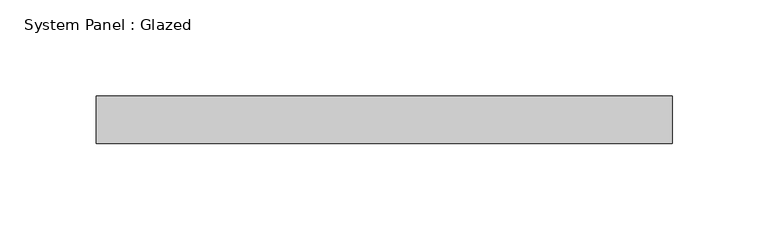
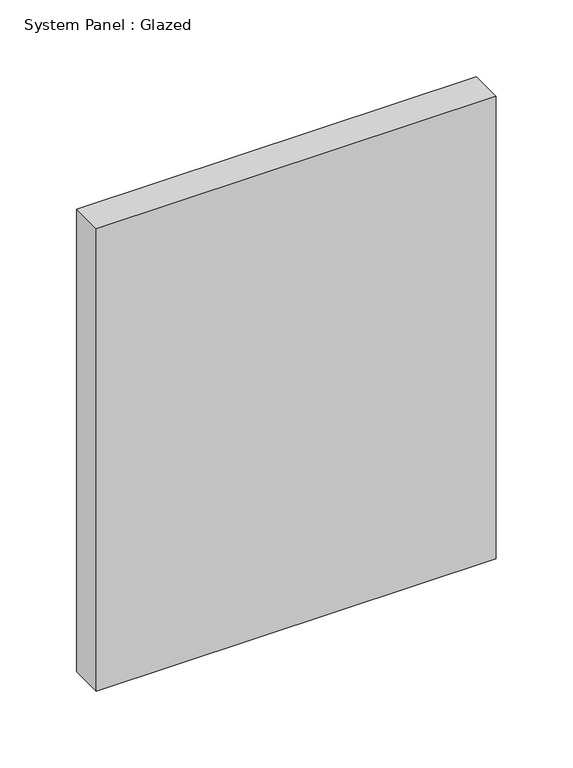
"""IFC4 building model written with IfcOpenShell, lengths in millimetres: plate geometry, System Panel : Glazed."""

import ifcopenshell
import ifcopenshell.guid

model = None  # the IFC model being written
_history = None  # IfcOwnerHistory: only IFC2X3 demands one
_inside = {}  # id of a spatial element -> (the spatial element, [elements in it])
_under = {}  # id of a project, library or spatial element -> (it, [spatial elements below it])
_declared = {}  # id of a project -> (the project, [libraries it declares])
_typed = {}  # id of a type object -> (the type object, [elements of that type])
_made_of = {}  # id of a material, layer set ... -> (it, [elements and type objects made of it])


def new_model(schema):
    """Start an empty IFC model of exactly this schema.

    Asked for "IFC4X3", IfcOpenShell would pick the latest addendum, in which some entities
    have other attributes; the version numbers below select the first issue.
    IFC2X3 requires an IfcOwnerHistory on every rooted entity: one is made here for all.
    """
    global model, _history
    if schema == "IFC4X3":
        model = ifcopenshell.file(schema_version=(4, 3, 0, 0))
    else:
        model = ifcopenshell.file(schema=schema)
    _inside.clear()
    _under.clear()
    _declared.clear()
    _typed.clear()
    _made_of.clear()
    _history = None
    if model.schema == "IFC2X3":
        org = make("IfcOrganization", Name="unknown")
        user = make(
            "IfcPersonAndOrganization",
            ThePerson=make("IfcPerson", FamilyName="unknown"),
            TheOrganization=org,
        )
        app = make(
            "IfcApplication",
            ApplicationDeveloper=org,
            Version="unknown",
            ApplicationFullName="unknown",
            ApplicationIdentifier="unknown",
        )
        _history = make(
            "IfcOwnerHistory",
            OwningUser=user,
            OwningApplication=app,
            ChangeAction="ADDED",
            CreationDate=0,
        )
    return model


def make(cls, **values):
    """One entity of the class cls with the attributes given. An attribute that is None is left unset."""
    return model.create_entity(
        cls, **{name: value for name, value in values.items() if value is not None}
    )


def rooted(cls, **values):
    """An entity with a GlobalId (a new one), such as an element, a storey or a relation."""
    return make(cls, GlobalId=ifcopenshell.guid.new(), OwnerHistory=_history, **values)


def si_unit(unit_type, name, prefix=None):
    """IfcSIUnit, for example si_unit("LENGTHUNIT", "METRE", prefix="MILLI")."""
    return make("IfcSIUnit", UnitType=unit_type, Prefix=prefix, Name=name)


def assignment(units):
    """IfcUnitAssignment: the units of a project."""
    return None if units is None else make("IfcUnitAssignment", Units=units)


def point(xyz):
    """IfcCartesianPoint."""
    return None if xyz is None else make("IfcCartesianPoint", Coordinates=xyz)


def direction(xyz):
    """IfcDirection."""
    return None if xyz is None else make("IfcDirection", DirectionRatios=xyz)


def frame(location, z_axis=None, x_axis=None):
    """IfcAxis2Placement3D, a coordinate frame: its origin and axes. An axis left out is left unset."""
    return make(
        "IfcAxis2Placement3D",
        Location=point(location),
        Axis=direction(z_axis),
        RefDirection=direction(x_axis),
    )


def origin():
    """The frame at (0, 0, 0) with its axes left unset."""
    return frame((0.0, 0.0, 0.0))


def origin_with_axes():
    """The frame at (0, 0, 0) with the z axis (0, 0, 1) and the x axis (1, 0, 0) written out."""
    return frame((0.0, 0.0, 0.0), z_axis=(0.0, 0.0, 1.0), x_axis=(1.0, 0.0, 0.0))


def place(relative_to, where):
    """IfcLocalPlacement: puts the frame where relative to a parent placement (None: the world)."""
    return make(
        "IfcLocalPlacement", PlacementRelTo=relative_to, RelativePlacement=where
    )


def context(
    kind, dimensions, precision=None, world=None, true_north=None, identifier=None
):
    """IfcGeometricRepresentationContext, for example the 3D "Model" context."""
    return make(
        "IfcGeometricRepresentationContext",
        ContextIdentifier=identifier,
        ContextType=kind,
        CoordinateSpaceDimension=dimensions,
        Precision=precision,
        WorldCoordinateSystem=world,
        TrueNorth=true_north,
    )


def project(units=None, contexts=None):
    """IfcProject with its units and contexts."""
    return rooted(
        "IfcProject",
        Name="project",
        RepresentationContexts=contexts,
        UnitsInContext=assignment(units),
    )


def spatial(cls, under=None, at=None, **own):
    """A site, building, storey or space (cls), placed at a placement, below another one or the project."""
    s = rooted(cls, ObjectPlacement=at, **own)
    if under is not None:
        _under.setdefault(under.id(), (under, []))[1].append(s)
    return s


def polyline(points):
    """IfcPolyline through the points."""
    return make("IfcPolyline", Points=[point(p) for p in points])


def outline(outer, holes=None, kind="AREA"):
    """IfcArbitraryClosedProfileDef: a profile drawn as a closed curve; with holes, ...WithVoids."""
    if holes is None:
        return make("IfcArbitraryClosedProfileDef", ProfileType=kind, OuterCurve=outer)
    return make(
        "IfcArbitraryProfileDefWithVoids",
        ProfileType=kind,
        OuterCurve=outer,
        InnerCurves=holes,
    )


def extrude(swept, where, along, depth):
    """IfcExtrudedAreaSolid: the profile swept, set in the frame where, extruded along a direction by depth."""
    return make(
        "IfcExtrudedAreaSolid",
        SweptArea=swept,
        Position=where,
        ExtrudedDirection=direction(along),
        Depth=depth,
    )


def shape(context_of_items, identifier, shape_type, items):
    """IfcShapeRepresentation: the items that make up one representation, for example the "Body"."""
    return make(
        "IfcShapeRepresentation",
        ContextOfItems=context_of_items,
        RepresentationIdentifier=identifier,
        RepresentationType=shape_type,
        Items=items,
    )


def source(mapping_origin, context_of_items, identifier, shape_type, items):
    """IfcRepresentationMap: a shape defined once, which mapped items show again and again."""
    return make(
        "IfcRepresentationMap",
        MappingOrigin=mapping_origin,
        MappedRepresentation=shape(context_of_items, identifier, shape_type, items),
    )


def transform(
    local_origin,
    x_axis=None,
    y_axis=None,
    z_axis=None,
    scale=None,
    scale2=None,
    scale3=None,
    uniform=True,
):
    """IfcCartesianTransformationOperator3D, or its non-uniform kind. x_axis, y_axis, z_axis: its Axis1, 2, 3."""
    if uniform:
        return make(
            "IfcCartesianTransformationOperator3D",
            Axis1=direction(x_axis),
            Axis2=direction(y_axis),
            LocalOrigin=point(local_origin),
            Scale=scale,
            Axis3=direction(z_axis),
        )
    return make(
        "IfcCartesianTransformationOperator3DnonUniform",
        Axis1=direction(x_axis),
        Axis2=direction(y_axis),
        LocalOrigin=point(local_origin),
        Scale=scale,
        Axis3=direction(z_axis),
        Scale2=scale2,
        Scale3=scale3,
    )


def mapped(mapping_source, mapping_target):
    """IfcMappedItem: shows the shape of a source again, moved by a transform."""
    return make(
        "IfcMappedItem", MappingSource=mapping_source, MappingTarget=mapping_target
    )


def made_of(thing, what):
    """Note that an element or type object is made of a material, layer set ...; save() writes the relation."""
    if what is not None:
        _made_of.setdefault(what.id(), (what, []))[1].append(thing)
    return thing


def element(
    cls,
    number,
    at=None,
    inside=None,
    cuts=None,
    type_object=None,
    material=None,
    context=None,
    identifier="Body",
    shape_type=None,
    held_by="IfcProductDefinitionShape",
    body=None,
    shapes=None,
    **own,
):
    """One element of the class cls, such as IfcWall. Its Tag is "e" and its number.

    at: its placement. inside: the storey or other place that contains it. cuts: it is an
    opening in that element (IfcRelVoidsElement). A single representation is given by context,
    identifier, shape_type and body (its items); several are given by shapes. held_by: the class
    of the entity that holds the representations. save() writes the other relations.
    """
    e = rooted(cls, Tag="e%d" % number, ObjectPlacement=at, **own)
    if body is not None:
        shapes = [shape(context, identifier, shape_type, body)]
    if shapes is not None:
        e.Representation = make(held_by, Representations=shapes)
    if inside is not None:
        _inside.setdefault(inside.id(), (inside, []))[1].append(e)
    if cuts is not None:
        rooted(
            "IfcRelVoidsElement", RelatingBuildingElement=cuts, RelatedOpeningElement=e
        )
    if type_object is not None:
        _typed.setdefault(type_object.id(), (type_object, []))[1].append(e)
    return made_of(e, material)


def aggregate(whole, parts):
    """IfcRelAggregates: a whole, such as a stair, and the parts it consists of."""
    return rooted("IfcRelAggregates", RelatingObject=whole, RelatedObjects=parts)


def save(model, path):
    """Write the relations noted so far, then the file.

    IfcRelAggregates (storeys below a building ...), IfcRelContainedInSpatialStructure (elements
    in a storey), IfcRelDefinesByType, IfcRelAssociatesMaterial and IfcRelDeclares: one each for
    every whole, place, type object, material and project.
    """
    for whole, parts in _under.values():
        aggregate(whole, parts)
    for where, things in _inside.values():
        rooted(
            "IfcRelContainedInSpatialStructure",
            RelatedElements=things,
            RelatingStructure=where,
        )
    for kind, things in _typed.values():
        rooted("IfcRelDefinesByType", RelatedObjects=things, RelatingType=kind)
    for what, things in _made_of.values():
        rooted("IfcRelAssociatesMaterial", RelatedObjects=things, RelatingMaterial=what)
    for by, libraries in _declared.values():
        rooted("IfcRelDeclares", RelatingContext=by, RelatedDefinitions=libraries)
    model.write(path)


def system_panel_glazed_74f4a765(model_context):
    return source(origin(), model_context, "Body", "SweptSolid", [
        extrude(outline(polyline([(150.0, 24.5), (-150.0, 24.5), (-150.0, 49.5), (150.0, 49.5), (150.0, 24.5)])), origin_with_axes(), (0.0, 0.0, 1.0), 366.6666667),
    ])


if __name__ == "__main__":
    model = new_model("IFC4")
    model_context = context("Model", 3, world=origin())
    ifc_project = project(units=[si_unit("LENGTHUNIT", "METRE", prefix="MILLI")], contexts=[model_context])
    site = spatial("IfcSite", under=ifc_project)
    building = spatial("IfcBuilding", under=site)
    placement = place(None, origin())
    system_panel_glazed_shape = system_panel_glazed_74f4a765(model_context)
    element("IfcPlate", 1, ObjectType="System Panel : Glazed", at=placement, inside=building, context=model_context, shape_type="MappedRepresentation", body=[
        mapped(system_panel_glazed_shape, transform((0.0, 0.0, 0.0), x_axis=(1.0, 0.0, 0.0), y_axis=(0.0, 1.0, 0.0), z_axis=(0.0, 0.0, 1.0))),
    ])
    save(model, "model.ifc")

# Revit data of these elements
# Element 1 (IfcPlate, "System Panel : Glazed")
#   Materials on its faces: "Glass"
# Materials
#   "Glass": class "Glass", colour RGB 218 227 224, transparency 0.85, Description = "Soda Lime Glass", Cost = 0
